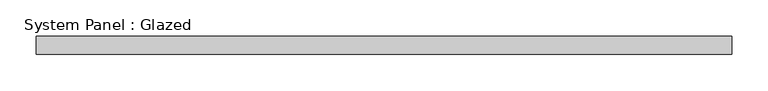
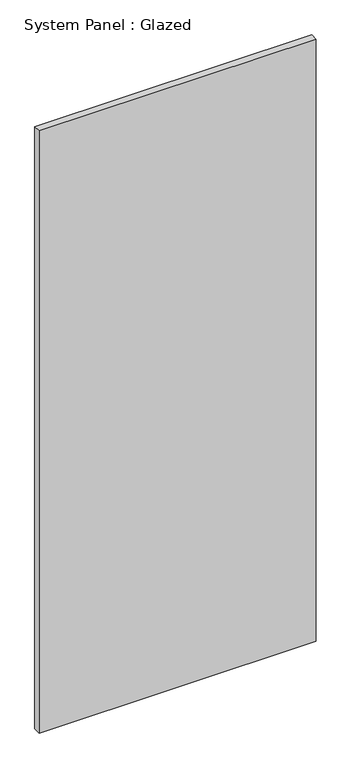
"""IFC4 building model written with IfcOpenShell, lengths in millimetres: plate geometry, System Panel : Glazed."""

import ifcopenshell
import ifcopenshell.guid

model = None  # the IFC model being written
_history = None  # IfcOwnerHistory: only IFC2X3 demands one
_inside = {}  # id of a spatial element -> (the spatial element, [elements in it])
_under = {}  # id of a project, library or spatial element -> (it, [spatial elements below it])
_declared = {}  # id of a project -> (the project, [libraries it declares])
_typed = {}  # id of a type object -> (the type object, [elements of that type])
_made_of = {}  # id of a material, layer set ... -> (it, [elements and type objects made of it])


def new_model(schema):
    """Start an empty IFC model of exactly this schema.

    Asked for "IFC4X3", IfcOpenShell would pick the latest addendum, in which some entities
    have other attributes; the version numbers below select the first issue.
    IFC2X3 requires an IfcOwnerHistory on every rooted entity: one is made here for all.
    """
    global model, _history
    if schema == "IFC4X3":
        model = ifcopenshell.file(schema_version=(4, 3, 0, 0))
    else:
        model = ifcopenshell.file(schema=schema)
    _inside.clear()
    _under.clear()
    _declared.clear()
    _typed.clear()
    _made_of.clear()
    _history = None
    if model.schema == "IFC2X3":
        org = make("IfcOrganization", Name="unknown")
        user = make(
            "IfcPersonAndOrganization",
            ThePerson=make("IfcPerson", FamilyName="unknown"),
            TheOrganization=org,
        )
        app = make(
            "IfcApplication",
            ApplicationDeveloper=org,
            Version="unknown",
            ApplicationFullName="unknown",
            ApplicationIdentifier="unknown",
        )
        _history = make(
            "IfcOwnerHistory",
            OwningUser=user,
            OwningApplication=app,
            ChangeAction="ADDED",
            CreationDate=0,
        )
    return model


def make(cls, **values):
    """One entity of the class cls with the attributes given. An attribute that is None is left unset."""
    return model.create_entity(
        cls, **{name: value for name, value in values.items() if value is not None}
    )


def rooted(cls, **values):
    """An entity with a GlobalId (a new one), such as an element, a storey or a relation."""
    return make(cls, GlobalId=ifcopenshell.guid.new(), OwnerHistory=_history, **values)


def si_unit(unit_type, name, prefix=None):
    """IfcSIUnit, for example si_unit("LENGTHUNIT", "METRE", prefix="MILLI")."""
    return make("IfcSIUnit", UnitType=unit_type, Prefix=prefix, Name=name)


def assignment(units):
    """IfcUnitAssignment: the units of a project."""
    return None if units is None else make("IfcUnitAssignment", Units=units)


def point(xyz):
    """IfcCartesianPoint."""
    return None if xyz is None else make("IfcCartesianPoint", Coordinates=xyz)


def direction(xyz):
    """IfcDirection."""
    return None if xyz is None else make("IfcDirection", DirectionRatios=xyz)


def frame(location, z_axis=None, x_axis=None):
    """IfcAxis2Placement3D, a coordinate frame: its origin and axes. An axis left out is left unset."""
    return make(
        "IfcAxis2Placement3D",
        Location=point(location),
        Axis=direction(z_axis),
        RefDirection=direction(x_axis),
    )


def origin():
    """The frame at (0, 0, 0) with its axes left unset."""
    return frame((0.0, 0.0, 0.0))


def origin_with_axes():
    """The frame at (0, 0, 0) with the z axis (0, 0, 1) and the x axis (1, 0, 0) written out."""
    return frame((0.0, 0.0, 0.0), z_axis=(0.0, 0.0, 1.0), x_axis=(1.0, 0.0, 0.0))


def place(relative_to, where):
    """IfcLocalPlacement: puts the frame where relative to a parent placement (None: the world)."""
    return make(
        "IfcLocalPlacement", PlacementRelTo=relative_to, RelativePlacement=where
    )


def context(
    kind, dimensions, precision=None, world=None, true_north=None, identifier=None
):
    """IfcGeometricRepresentationContext, for example the 3D "Model" context."""
    return make(
        "IfcGeometricRepresentationContext",
        ContextIdentifier=identifier,
        ContextType=kind,
        CoordinateSpaceDimension=dimensions,
        Precision=precision,
        WorldCoordinateSystem=world,
        TrueNorth=true_north,
    )


def project(units=None, contexts=None):
    """IfcProject with its units and contexts."""
    return rooted(
        "IfcProject",
        Name="project",
        RepresentationContexts=contexts,
        UnitsInContext=assignment(units),
    )


def spatial(cls, under=None, at=None, **own):
    """A site, building, storey or space (cls), placed at a placement, below another one or the project."""
    s = rooted(cls, ObjectPlacement=at, **own)
    if under is not None:
        _under.setdefault(under.id(), (under, []))[1].append(s)
    return s


def polyline(points):
    """IfcPolyline through the points."""
    return make("IfcPolyline", Points=[point(p) for p in points])


def outline(outer, holes=None, kind="AREA"):
    """IfcArbitraryClosedProfileDef: a profile drawn as a closed curve; with holes, ...WithVoids."""
    if holes is None:
        return make("IfcArbitraryClosedProfileDef", ProfileType=kind, OuterCurve=outer)
    return make(
        "IfcArbitraryProfileDefWithVoids",
        ProfileType=kind,
        OuterCurve=outer,
        InnerCurves=holes,
    )


def extrude(swept, where, along, depth):
    """IfcExtrudedAreaSolid: the profile swept, set in the frame where, extruded along a direction by depth."""
    return make(
        "IfcExtrudedAreaSolid",
        SweptArea=swept,
        Position=where,
        ExtrudedDirection=direction(along),
        Depth=depth,
    )


def shape(context_of_items, identifier, shape_type, items):
    """IfcShapeRepresentation: the items that make up one representation, for example the "Body"."""
    return make(
        "IfcShapeRepresentation",
        ContextOfItems=context_of_items,
        RepresentationIdentifier=identifier,
        RepresentationType=shape_type,
        Items=items,
    )


def source(mapping_origin, context_of_items, identifier, shape_type, items):
    """IfcRepresentationMap: a shape defined once, which mapped items show again and again."""
    return make(
        "IfcRepresentationMap",
        MappingOrigin=mapping_origin,
        MappedRepresentation=shape(context_of_items, identifier, shape_type, items),
    )


def transform(
    local_origin,
    x_axis=None,
    y_axis=None,
    z_axis=None,
    scale=None,
    scale2=None,
    scale3=None,
    uniform=True,
):
    """IfcCartesianTransformationOperator3D, or its non-uniform kind. x_axis, y_axis, z_axis: its Axis1, 2, 3."""
    if uniform:
        return make(
            "IfcCartesianTransformationOperator3D",
            Axis1=direction(x_axis),
            Axis2=direction(y_axis),
            LocalOrigin=point(local_origin),
            Scale=scale,
            Axis3=direction(z_axis),
        )
    return make(
        "IfcCartesianTransformationOperator3DnonUniform",
        Axis1=direction(x_axis),
        Axis2=direction(y_axis),
        LocalOrigin=point(local_origin),
        Scale=scale,
        Axis3=direction(z_axis),
        Scale2=scale2,
        Scale3=scale3,
    )


def mapped(mapping_source, mapping_target):
    """IfcMappedItem: shows the shape of a source again, moved by a transform."""
    return make(
        "IfcMappedItem", MappingSource=mapping_source, MappingTarget=mapping_target
    )


def made_of(thing, what):
    """Note that an element or type object is made of a material, layer set ...; save() writes the relation."""
    if what is not None:
        _made_of.setdefault(what.id(), (what, []))[1].append(thing)
    return thing


def element(
    cls,
    number,
    at=None,
    inside=None,
    cuts=None,
    type_object=None,
    material=None,
    context=None,
    identifier="Body",
    shape_type=None,
    held_by="IfcProductDefinitionShape",
    body=None,
    shapes=None,
    **own,
):
    """One element of the class cls, such as IfcWall. Its Tag is "e" and its number.

    at: its placement. inside: the storey or other place that contains it. cuts: it is an
    opening in that element (IfcRelVoidsElement). A single representation is given by context,
    identifier, shape_type and body (its items); several are given by shapes. held_by: the class
    of the entity that holds the representations. save() writes the other relations.
    """
    e = rooted(cls, Tag="e%d" % number, ObjectPlacement=at, **own)
    if body is not None:
        shapes = [shape(context, identifier, shape_type, body)]
    if shapes is not None:
        e.Representation = make(held_by, Representations=shapes)
    if inside is not None:
        _inside.setdefault(inside.id(), (inside, []))[1].append(e)
    if cuts is not None:
        rooted(
            "IfcRelVoidsElement", RelatingBuildingElement=cuts, RelatedOpeningElement=e
        )
    if type_object is not None:
        _typed.setdefault(type_object.id(), (type_object, []))[1].append(e)
    return made_of(e, material)


def aggregate(whole, parts):
    """IfcRelAggregates: a whole, such as a stair, and the parts it consists of."""
    return rooted("IfcRelAggregates", RelatingObject=whole, RelatedObjects=parts)


def save(model, path):
    """Write the relations noted so far, then the file.

    IfcRelAggregates (storeys below a building ...), IfcRelContainedInSpatialStructure (elements
    in a storey), IfcRelDefinesByType, IfcRelAssociatesMaterial and IfcRelDeclares: one each for
    every whole, place, type object, material and project.
    """
    for whole, parts in _under.values():
        aggregate(whole, parts)
    for where, things in _inside.values():
        rooted(
            "IfcRelContainedInSpatialStructure",
            RelatedElements=things,
            RelatingStructure=where,
        )
    for kind, things in _typed.values():
        rooted("IfcRelDefinesByType", RelatedObjects=things, RelatingType=kind)
    for what, things in _made_of.values():
        rooted("IfcRelAssociatesMaterial", RelatedObjects=things, RelatingMaterial=what)
    for by, libraries in _declared.values():
        rooted("IfcRelDeclares", RelatingContext=by, RelatedDefinitions=libraries)
    model.write(path)


def system_panel_glazed_8c511674(model_context):
    return source(origin(), model_context, "Body", "SweptSolid", [
        extrude(outline(polyline([(482.5999999, -44.45), (-482.5999999, -44.45), (-482.5999999, -19.05), (482.5999999, -19.05), (482.5999999, -44.45)])), origin_with_axes(), (0.0, 0.0, 1.0), 2216.15),
    ])


if __name__ == "__main__":
    model = new_model("IFC4")
    model_context = context("Model", 3, world=origin())
    ifc_project = project(units=[si_unit("LENGTHUNIT", "METRE", prefix="MILLI")], contexts=[model_context])
    site = spatial("IfcSite", under=ifc_project)
    building = spatial("IfcBuilding", under=site)
    placement = place(None, origin())
    system_panel_glazed_shape = system_panel_glazed_8c511674(model_context)
    element("IfcPlate", 1, ObjectType="System Panel : Glazed", at=placement, inside=building, context=model_context, shape_type="MappedRepresentation", body=[
        mapped(system_panel_glazed_shape, transform((0.0, 0.0, 0.0), x_axis=(1.0, 0.0, 0.0), y_axis=(0.0, 1.0, 0.0), z_axis=(0.0, 0.0, 1.0))),
    ])
    save(model, "model.ifc")

# Revit data of these elements
# Type "System Panel : Glazed"
#   Construction Type Id = "GSP4R"
#   Analytic Construction = "1/8 in Pilkington single glazing"
#   Visual Light Transmittance = 0.9
#   Solar Heat Gain Coefficient = 0.86
#   Heat Transfer Coefficient (U) = 1.18115 BTU/(h·ft²·°F)
#   Define Thermal Properties by = 1
# Element 1 (IfcPlate, "System Panel : Glazed")
#   Materials on its faces: "Glass"
# Materials
#   "Glass": class "Glass", colour RGB 0 128 192, transparency 0.75, Description = "Soda Lime Glass", Cost = 0
